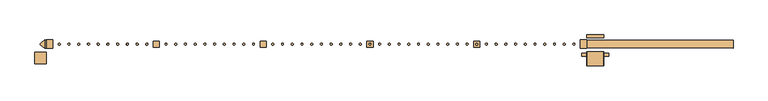
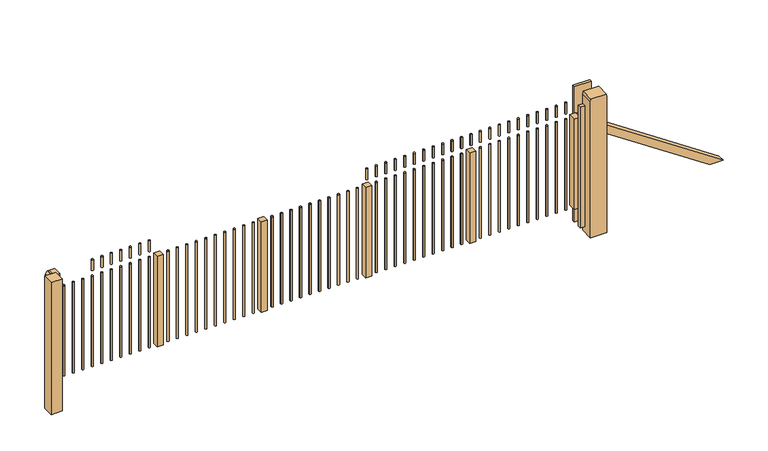
"""IFC4 building model written with IfcOpenShell, lengths in millimetres: door geometry, NLRS_90_DO_UN_schuifpoort met spijlen_gen_rsf : schuifpoort automatisch bxh 7000x1800-NP."""

from ifc_helpers import new_model, si_unit, point, frame, frame_2d, origin, place, context, project, spatial, polyline, circle_curve, trimmed, segment, composite_curve, outline, extrude, source, transform, mapped, element, save


def door_c2b4a2f6(model_context):
    return source(origin(), model_context, "Body", "SweptSolid", [
        extrude(outline(composite_curve([segment(trimmed(circle_curve(frame_2d((3299.5, 0.0)), 12.5), [point((3312.0, 0.0))], [point((3287.0, 0.0))], False, "CARTESIAN"), True, "CONTINUOUS"), segment(trimmed(circle_curve(frame_2d((3299.5, 0.0)), 12.5), [point((3287.0, 0.0))], [point((3312.0, 0.0))], False, "CARTESIAN"), True, "CONTINUOUS")], self_intersect=False)), frame((0.0, 0.0, 300.0), z_axis=(0.0, 0.0, 1.0), x_axis=(1.0, 0.0, 0.0)), (0.0, 0.0, 1.0), 1270.0),
        extrude(outline(composite_curve([segment(trimmed(circle_curve(frame_2d((3173.5, 0.0)), 12.5), [point((3186.0, 0.0))], [point((3161.0, 0.0))], False, "CARTESIAN"), True, "CONTINUOUS"), segment(trimmed(circle_curve(frame_2d((3173.5, 0.0)), 12.5), [point((3161.0, 0.0))], [point((3186.0, 0.0))], False, "CARTESIAN"), True, "CONTINUOUS")], self_intersect=False)), frame((0.0, 0.0, 300.0), z_axis=(0.0, 0.0, 1.0), x_axis=(1.0, 0.0, 0.0)), (0.0, 0.0, 1.0), 1270.0),
        extrude(outline(composite_curve([segment(trimmed(circle_curve(frame_2d((3047.5, 0.0)), 12.5), [point((3060.0, 0.0))], [point((3035.0, 0.0))], False, "CARTESIAN"), True, "CONTINUOUS"), segment(trimmed(circle_curve(frame_2d((3047.5, 0.0)), 12.5), [point((3035.0, 0.0))], [point((3060.0, 0.0))], False, "CARTESIAN"), True, "CONTINUOUS")], self_intersect=False)), frame((0.0, 0.0, 300.0), z_axis=(0.0, 0.0, 1.0), x_axis=(1.0, 0.0, 0.0)), (0.0, 0.0, 1.0), 1270.0),
        extrude(outline(composite_curve([segment(trimmed(circle_curve(frame_2d((2921.5, 0.0)), 12.5), [point((2934.0, 0.0))], [point((2909.0, 0.0))], False, "CARTESIAN"), True, "CONTINUOUS"), segment(trimmed(circle_curve(frame_2d((2921.5, 0.0)), 12.5), [point((2909.0, 0.0))], [point((2934.0, 0.0))], False, "CARTESIAN"), True, "CONTINUOUS")], self_intersect=False)), frame((0.0, 0.0, 300.0), z_axis=(0.0, 0.0, 1.0), x_axis=(1.0, 0.0, 0.0)), (0.0, 0.0, 1.0), 1270.0),
        extrude(outline(composite_curve([segment(trimmed(circle_curve(frame_2d((2795.5, 0.0)), 12.5), [point((2808.0, 0.0))], [point((2783.0, 0.0))], False, "CARTESIAN"), True, "CONTINUOUS"), segment(trimmed(circle_curve(frame_2d((2795.5, 0.0)), 12.5), [point((2783.0, 0.0))], [point((2808.0, 0.0))], False, "CARTESIAN"), True, "CONTINUOUS")], self_intersect=False)), frame((0.0, 0.0, 300.0), z_axis=(0.0, 0.0, 1.0), x_axis=(1.0, 0.0, 0.0)), (0.0, 0.0, 1.0), 1270.0),
        extrude(outline(composite_curve([segment(trimmed(circle_curve(frame_2d((2669.5, 0.0)), 12.5), [point((2682.0, 0.0))], [point((2657.0, 0.0))], False, "CARTESIAN"), True, "CONTINUOUS"), segment(trimmed(circle_curve(frame_2d((2669.5, 0.0)), 12.5), [point((2657.0, 0.0))], [point((2682.0, 0.0))], False, "CARTESIAN"), True, "CONTINUOUS")], self_intersect=False)), frame((0.0, 0.0, 300.0), z_axis=(0.0, 0.0, 1.0), x_axis=(1.0, 0.0, 0.0)), (0.0, 0.0, 1.0), 1270.0),
        extrude(outline(composite_curve([segment(trimmed(circle_curve(frame_2d((2543.5, 0.0)), 12.5), [point((2556.0, 0.0))], [point((2531.0, 0.0))], False, "CARTESIAN"), True, "CONTINUOUS"), segment(trimmed(circle_curve(frame_2d((2543.5, 0.0)), 12.5), [point((2531.0, 0.0))], [point((2556.0, 0.0))], False, "CARTESIAN"), True, "CONTINUOUS")], self_intersect=False)), frame((0.0, 0.0, 300.0), z_axis=(0.0, 0.0, 1.0), x_axis=(1.0, 0.0, 0.0)), (0.0, 0.0, 1.0), 1270.0),
        extrude(outline(composite_curve([segment(trimmed(circle_curve(frame_2d((2417.5, 0.0)), 12.5), [point((2430.0, 0.0))], [point((2405.0, 0.0))], False, "CARTESIAN"), True, "CONTINUOUS"), segment(trimmed(circle_curve(frame_2d((2417.5, 0.0)), 12.5), [point((2405.0, 0.0))], [point((2430.0, 0.0))], False, "CARTESIAN"), True, "CONTINUOUS")], self_intersect=False)), frame((0.0, 0.0, 300.0), z_axis=(0.0, 0.0, 1.0), x_axis=(1.0, 0.0, 0.0)), (0.0, 0.0, 1.0), 1270.0),
        extrude(outline(composite_curve([segment(trimmed(circle_curve(frame_2d((2291.5, 0.0)), 12.5), [point((2304.0, 0.0))], [point((2279.0, 0.0))], False, "CARTESIAN"), True, "CONTINUOUS"), segment(trimmed(circle_curve(frame_2d((2291.5, 0.0)), 12.5), [point((2279.0, 0.0))], [point((2304.0, 0.0))], False, "CARTESIAN"), True, "CONTINUOUS")], self_intersect=False)), frame((0.0, 0.0, 300.0), z_axis=(0.0, 0.0, 1.0), x_axis=(1.0, 0.0, 0.0)), (0.0, 0.0, 1.0), 1270.0),
        extrude(outline(composite_curve([segment(trimmed(circle_curve(frame_2d((2165.5, 0.0)), 12.5), [point((2178.0, 0.0))], [point((2153.0, 0.0))], False, "CARTESIAN"), True, "CONTINUOUS"), segment(trimmed(circle_curve(frame_2d((2165.5, 0.0)), 12.5), [point((2153.0, 0.0))], [point((2178.0, 0.0))], False, "CARTESIAN"), True, "CONTINUOUS")], self_intersect=False)), frame((0.0, 0.0, 300.0), z_axis=(0.0, 0.0, 1.0), x_axis=(1.0, 0.0, 0.0)), (0.0, 0.0, 1.0), 1270.0),
        extrude(outline(composite_curve([segment(trimmed(circle_curve(frame_2d((1915.5, 0.0)), 12.5), [point((1928.0, 0.0))], [point((1903.0, 0.0))], False, "CARTESIAN"), True, "CONTINUOUS"), segment(trimmed(circle_curve(frame_2d((1915.5, 0.0)), 12.5), [point((1903.0, 0.0))], [point((1928.0, 0.0))], False, "CARTESIAN"), True, "CONTINUOUS")], self_intersect=False)), frame((0.0, 0.0, 300.0), z_axis=(0.0, 0.0, 1.0), x_axis=(1.0, 0.0, 0.0)), (0.0, 0.0, 1.0), 1270.0),
        extrude(outline(composite_curve([segment(trimmed(circle_curve(frame_2d((1789.5, 0.0)), 12.5), [point((1802.0, 0.0))], [point((1777.0, 0.0))], False, "CARTESIAN"), True, "CONTINUOUS"), segment(trimmed(circle_curve(frame_2d((1789.5, 0.0)), 12.5), [point((1777.0, 0.0))], [point((1802.0, 0.0))], False, "CARTESIAN"), True, "CONTINUOUS")], self_intersect=False)), frame((0.0, 0.0, 300.0), z_axis=(0.0, 0.0, 1.0), x_axis=(1.0, 0.0, 0.0)), (0.0, 0.0, 1.0), 1270.0),
        extrude(outline(composite_curve([segment(trimmed(circle_curve(frame_2d((1663.5, 0.0)), 12.5), [point((1676.0, 0.0))], [point((1651.0, 0.0))], False, "CARTESIAN"), True, "CONTINUOUS"), segment(trimmed(circle_curve(frame_2d((1663.5, 0.0)), 12.5), [point((1651.0, 0.0))], [point((1676.0, 0.0))], False, "CARTESIAN"), True, "CONTINUOUS")], self_intersect=False)), frame((0.0, 0.0, 300.0), z_axis=(0.0, 0.0, 1.0), x_axis=(1.0, 0.0, 0.0)), (0.0, 0.0, 1.0), 1270.0),
        extrude(outline(composite_curve([segment(trimmed(circle_curve(frame_2d((1537.5, 0.0)), 12.5), [point((1550.0, 0.0))], [point((1525.0, 0.0))], False, "CARTESIAN"), True, "CONTINUOUS"), segment(trimmed(circle_curve(frame_2d((1537.5, 0.0)), 12.5), [point((1525.0, 0.0))], [point((1550.0, 0.0))], False, "CARTESIAN"), True, "CONTINUOUS")], self_intersect=False)), frame((0.0, 0.0, 300.0), z_axis=(0.0, 0.0, 1.0), x_axis=(1.0, 0.0, 0.0)), (0.0, 0.0, 1.0), 1270.0),
        extrude(outline(composite_curve([segment(trimmed(circle_curve(frame_2d((1411.5, 0.0)), 12.5), [point((1424.0, 0.0))], [point((1399.0, 0.0))], False, "CARTESIAN"), True, "CONTINUOUS"), segment(trimmed(circle_curve(frame_2d((1411.5, 0.0)), 12.5), [point((1399.0, 0.0))], [point((1424.0, 0.0))], False, "CARTESIAN"), True, "CONTINUOUS")], self_intersect=False)), frame((0.0, 0.0, 300.0), z_axis=(0.0, 0.0, 1.0), x_axis=(1.0, 0.0, 0.0)), (0.0, 0.0, 1.0), 1270.0),
        extrude(outline(composite_curve([segment(trimmed(circle_curve(frame_2d((1285.5, 0.0)), 12.5), [point((1298.0, 0.0))], [point((1273.0, 0.0))], False, "CARTESIAN"), True, "CONTINUOUS"), segment(trimmed(circle_curve(frame_2d((1285.5, 0.0)), 12.5), [point((1273.0, 0.0))], [point((1298.0, 0.0))], False, "CARTESIAN"), True, "CONTINUOUS")], self_intersect=False)), frame((0.0, 0.0, 300.0), z_axis=(0.0, 0.0, 1.0), x_axis=(1.0, 0.0, 0.0)), (0.0, 0.0, 1.0), 1270.0),
        extrude(outline(composite_curve([segment(trimmed(circle_curve(frame_2d((1159.5, 0.0)), 12.5), [point((1172.0, 0.0))], [point((1147.0, 0.0))], False, "CARTESIAN"), True, "CONTINUOUS"), segment(trimmed(circle_curve(frame_2d((1159.5, 0.0)), 12.5), [point((1147.0, 0.0))], [point((1172.0, 0.0))], False, "CARTESIAN"), True, "CONTINUOUS")], self_intersect=False)), frame((0.0, 0.0, 300.0), z_axis=(0.0, 0.0, 1.0), x_axis=(1.0, 0.0, 0.0)), (0.0, 0.0, 1.0), 1270.0),
        extrude(outline(composite_curve([segment(trimmed(circle_curve(frame_2d((1033.5, 0.0)), 12.5), [point((1046.0, 0.0))], [point((1021.0, 0.0))], False, "CARTESIAN"), True, "CONTINUOUS"), segment(trimmed(circle_curve(frame_2d((1033.5, 0.0)), 12.5), [point((1021.0, 0.0))], [point((1046.0, 0.0))], False, "CARTESIAN"), True, "CONTINUOUS")], self_intersect=False)), frame((0.0, 0.0, 300.0), z_axis=(0.0, 0.0, 1.0), x_axis=(1.0, 0.0, 0.0)), (0.0, 0.0, 1.0), 1270.0),
        extrude(outline(composite_curve([segment(trimmed(circle_curve(frame_2d((907.5, 0.0)), 12.5), [point((920.0, 0.0))], [point((895.0, 0.0))], False, "CARTESIAN"), True, "CONTINUOUS"), segment(trimmed(circle_curve(frame_2d((907.5, 0.0)), 12.5), [point((895.0, 0.0))], [point((920.0, 0.0))], False, "CARTESIAN"), True, "CONTINUOUS")], self_intersect=False)), frame((0.0, 0.0, 300.0), z_axis=(0.0, 0.0, 1.0), x_axis=(1.0, 0.0, 0.0)), (0.0, 0.0, 1.0), 1270.0),
        extrude(outline(composite_curve([segment(trimmed(circle_curve(frame_2d((781.5, 0.0)), 12.5), [point((794.0, 0.0))], [point((769.0, 0.0))], False, "CARTESIAN"), True, "CONTINUOUS"), segment(trimmed(circle_curve(frame_2d((781.5, 0.0)), 12.5), [point((769.0, 0.0))], [point((794.0, 0.0))], False, "CARTESIAN"), True, "CONTINUOUS")], self_intersect=False)), frame((0.0, 0.0, 300.0), z_axis=(0.0, 0.0, 1.0), x_axis=(1.0, 0.0, 0.0)), (0.0, 0.0, 1.0), 1270.0),
        extrude(outline(polyline([(3465.0, -158.5), (3400.0, -158.5), (3400.0, -118.5), (3465.0, -118.5), (3465.0, -158.5)])), frame((0.0, 0.0, 100.0), z_axis=(0.0, 0.0, 1.0), x_axis=(1.0, 0.0, 0.0)), (0.0, 0.0, 1.0), 1700.0),
        extrude(outline(polyline([(3685.0, -158.5), (3685.0, -118.5), (3750.0, -118.5), (3750.0, -158.5), (3685.0, -158.5)])), frame((0.0, 0.0, 100.0), z_axis=(0.0, 0.0, 1.0), x_axis=(1.0, 0.0, 0.0)), (0.0, 0.0, 1.0), 1700.0),
        extrude(outline(polyline([(3685.0, 84.5), (3465.0, 84.5), (3465.0, 119.5), (3685.0, 119.5), (3685.0, 84.5)])), frame((0.0, 0.0, 12.0), z_axis=(0.0, 0.0, 1.0), x_axis=(1.0, 0.0, 0.0)), (0.0, 0.0, 1.0), 1906.0),
        extrude(outline(polyline([(1918.0, 3465.0), (12.0, 3465.0), (12.0, 3685.0), (1918.0, 3685.0), (1960.0, 3677.5), (1960.0, 3472.5), (1918.0, 3465.0)])), frame((0.0, -280.5, 0.0), z_axis=(0.0, 1.0, 0.0), x_axis=(0.0, 0.0, 1.0)), (0.0, 0.0, 1.0), 180.0),
        extrude(outline(polyline([(2000.5, -40.0), (2000.5, 40.0), (2080.5, 40.0), (2080.5, -40.0), (2000.5, -40.0)])), frame((0.0, 0.0, 300.0), z_axis=(0.0, 0.0, 1.0), x_axis=(1.0, 0.0, 0.0)), (0.0, 0.0, 1.0), 1270.0),
        extrude(outline(polyline([(616.5, -40.0), (616.5, 40.0), (696.5, 40.0), (696.5, -40.0), (616.5, -40.0)])), frame((0.0, 0.0, 300.0), z_axis=(0.0, 0.0, 1.0), x_axis=(1.0, 0.0, 0.0)), (0.0, 0.0, 1.0), 1270.0),
        extrude(outline(polyline([(-767.5, -40.0), (-767.5, 40.0), (-687.5, 40.0), (-687.5, -40.0), (-767.5, -40.0)])), frame((0.0, 0.0, 300.0), z_axis=(0.0, 0.0, 1.0), x_axis=(1.0, 0.0, 0.0)), (0.0, 0.0, 1.0), 1270.0),
        extrude(outline(polyline([(-2151.5, -40.0), (-2151.5, 40.0), (-2071.5, 40.0), (-2071.5, -40.0), (-2151.5, -40.0)])), frame((0.0, 0.0, 300.0), z_axis=(0.0, 0.0, 1.0), x_axis=(1.0, 0.0, 0.0)), (0.0, 0.0, 1.0), 1270.0),
        extrude(outline(composite_curve([segment(trimmed(circle_curve(frame_2d((531.5, 0.0)), 12.5), [point((544.0, 0.0))], [point((519.0, 0.0))], False, "CARTESIAN"), True, "CONTINUOUS"), segment(trimmed(circle_curve(frame_2d((531.5, 0.0)), 12.5), [point((519.0, 0.0))], [point((544.0, 0.0))], False, "CARTESIAN"), True, "CONTINUOUS")], self_intersect=False)), frame((0.0, 0.0, 300.0), z_axis=(0.0, 0.0, 1.0), x_axis=(1.0, 0.0, 0.0)), (0.0, 0.0, 1.0), 1270.0),
        extrude(outline(composite_curve([segment(trimmed(circle_curve(frame_2d((405.5, 0.0)), 12.5), [point((418.0, 0.0))], [point((393.0, 0.0))], False, "CARTESIAN"), True, "CONTINUOUS"), segment(trimmed(circle_curve(frame_2d((405.5, 0.0)), 12.5), [point((393.0, 0.0))], [point((418.0, 0.0))], False, "CARTESIAN"), True, "CONTINUOUS")], self_intersect=False)), frame((0.0, 0.0, 300.0), z_axis=(0.0, 0.0, 1.0), x_axis=(1.0, 0.0, 0.0)), (0.0, 0.0, 1.0), 1270.0),
        extrude(outline(composite_curve([segment(trimmed(circle_curve(frame_2d((279.5, 0.0)), 12.5), [point((292.0, 0.0))], [point((267.0, 0.0))], False, "CARTESIAN"), True, "CONTINUOUS"), segment(trimmed(circle_curve(frame_2d((279.5, 0.0)), 12.5), [point((267.0, 0.0))], [point((292.0, 0.0))], False, "CARTESIAN"), True, "CONTINUOUS")], self_intersect=False)), frame((0.0, 0.0, 300.0), z_axis=(0.0, 0.0, 1.0), x_axis=(1.0, 0.0, 0.0)), (0.0, 0.0, 1.0), 1270.0),
        extrude(outline(composite_curve([segment(trimmed(circle_curve(frame_2d((153.5, 0.0)), 12.5), [point((166.0, 0.0))], [point((141.0, 0.0))], False, "CARTESIAN"), True, "CONTINUOUS"), segment(trimmed(circle_curve(frame_2d((153.5, 0.0)), 12.5), [point((141.0, 0.0))], [point((166.0, 0.0))], False, "CARTESIAN"), True, "CONTINUOUS")], self_intersect=False)), frame((0.0, 0.0, 300.0), z_axis=(0.0, 0.0, 1.0), x_axis=(1.0, 0.0, 0.0)), (0.0, 0.0, 1.0), 1270.0),
        extrude(outline(composite_curve([segment(trimmed(circle_curve(frame_2d((27.5, 0.0)), 12.5), [point((40.0, 0.0))], [point((15.0, 0.0))], False, "CARTESIAN"), True, "CONTINUOUS"), segment(trimmed(circle_curve(frame_2d((27.5, 0.0)), 12.5), [point((15.0, 0.0))], [point((40.0, 0.0))], False, "CARTESIAN"), True, "CONTINUOUS")], self_intersect=False)), frame((0.0, 0.0, 300.0), z_axis=(0.0, 0.0, 1.0), x_axis=(1.0, 0.0, 0.0)), (0.0, 0.0, 1.0), 1270.0),
        extrude(outline(composite_curve([segment(trimmed(circle_curve(frame_2d((-98.5, 0.0)), 12.5), [point((-86.0, 0.0))], [point((-111.0, 0.0))], False, "CARTESIAN"), True, "CONTINUOUS"), segment(trimmed(circle_curve(frame_2d((-98.5, 0.0)), 12.5), [point((-111.0, 0.0))], [point((-86.0, 0.0))], False, "CARTESIAN"), True, "CONTINUOUS")], self_intersect=False)), frame((0.0, 0.0, 300.0), z_axis=(0.0, 0.0, 1.0), x_axis=(1.0, 0.0, 0.0)), (0.0, 0.0, 1.0), 1270.0),
        extrude(outline(composite_curve([segment(trimmed(circle_curve(frame_2d((-224.5, 0.0)), 12.5), [point((-212.0, 0.0))], [point((-237.0, 0.0))], False, "CARTESIAN"), True, "CONTINUOUS"), segment(trimmed(circle_curve(frame_2d((-224.5, 0.0)), 12.5), [point((-237.0, 0.0))], [point((-212.0, 0.0))], False, "CARTESIAN"), True, "CONTINUOUS")], self_intersect=False)), frame((0.0, 0.0, 300.0), z_axis=(0.0, 0.0, 1.0), x_axis=(1.0, 0.0, 0.0)), (0.0, 0.0, 1.0), 1270.0),
        extrude(outline(composite_curve([segment(trimmed(circle_curve(frame_2d((-350.5, 0.0)), 12.5), [point((-338.0, 0.0))], [point((-363.0, 0.0))], False, "CARTESIAN"), True, "CONTINUOUS"), segment(trimmed(circle_curve(frame_2d((-350.5, 0.0)), 12.5), [point((-363.0, 0.0))], [point((-338.0, 0.0))], False, "CARTESIAN"), True, "CONTINUOUS")], self_intersect=False)), frame((0.0, 0.0, 300.0), z_axis=(0.0, 0.0, 1.0), x_axis=(1.0, 0.0, 0.0)), (0.0, 0.0, 1.0), 1270.0),
        extrude(outline(composite_curve([segment(trimmed(circle_curve(frame_2d((-476.5, 0.0)), 12.5), [point((-464.0, 0.0))], [point((-489.0, 0.0))], False, "CARTESIAN"), True, "CONTINUOUS"), segment(trimmed(circle_curve(frame_2d((-476.5, 0.0)), 12.5), [point((-489.0, 0.0))], [point((-464.0, 0.0))], False, "CARTESIAN"), True, "CONTINUOUS")], self_intersect=False)), frame((0.0, 0.0, 300.0), z_axis=(0.0, 0.0, 1.0), x_axis=(1.0, 0.0, 0.0)), (0.0, 0.0, 1.0), 1270.0),
        extrude(outline(composite_curve([segment(trimmed(circle_curve(frame_2d((-602.5, 0.0)), 12.5), [point((-590.0, 0.0))], [point((-615.0, 0.0))], False, "CARTESIAN"), True, "CONTINUOUS"), segment(trimmed(circle_curve(frame_2d((-602.5, 0.0)), 12.5), [point((-615.0, 0.0))], [point((-590.0, 0.0))], False, "CARTESIAN"), True, "CONTINUOUS")], self_intersect=False)), frame((0.0, 0.0, 300.0), z_axis=(0.0, 0.0, 1.0), x_axis=(1.0, 0.0, 0.0)), (0.0, 0.0, 1.0), 1270.0),
        extrude(outline(polyline([(300.0, 5362.0), (1570.0, 3464.5), (1449.6685917, 3464.5), (300.0, 5182.2135061), (300.0, 5362.0)])), frame((0.0, -50.0, 0.0), z_axis=(0.0, 1.0, 0.0), x_axis=(0.0, 0.0, 1.0)), (0.0, 0.0, 1.0), 100.0),
        extrude(outline(composite_curve([segment(trimmed(circle_curve(frame_2d((-852.5, 0.0)), 12.5), [point((-840.0, 0.0))], [point((-865.0, 0.0))], False, "CARTESIAN"), True, "CONTINUOUS"), segment(trimmed(circle_curve(frame_2d((-852.5, 0.0)), 12.5), [point((-865.0, 0.0))], [point((-840.0, 0.0))], False, "CARTESIAN"), True, "CONTINUOUS")], self_intersect=False)), frame((0.0, 0.0, 300.0), z_axis=(0.0, 0.0, 1.0), x_axis=(1.0, 0.0, 0.0)), (0.0, 0.0, 1.0), 1270.0),
        extrude(outline(composite_curve([segment(trimmed(circle_curve(frame_2d((-978.5, 0.0)), 12.5), [point((-966.0, 0.0))], [point((-991.0, 0.0))], False, "CARTESIAN"), True, "CONTINUOUS"), segment(trimmed(circle_curve(frame_2d((-978.5, 0.0)), 12.5), [point((-991.0, 0.0))], [point((-966.0, 0.0))], False, "CARTESIAN"), True, "CONTINUOUS")], self_intersect=False)), frame((0.0, 0.0, 300.0), z_axis=(0.0, 0.0, 1.0), x_axis=(1.0, 0.0, 0.0)), (0.0, 0.0, 1.0), 1270.0),
        extrude(outline(composite_curve([segment(trimmed(circle_curve(frame_2d((-1104.5, 0.0)), 12.5), [point((-1092.0, 0.0))], [point((-1117.0, 0.0))], False, "CARTESIAN"), True, "CONTINUOUS"), segment(trimmed(circle_curve(frame_2d((-1104.5, 0.0)), 12.5), [point((-1117.0, 0.0))], [point((-1092.0, 0.0))], False, "CARTESIAN"), True, "CONTINUOUS")], self_intersect=False)), frame((0.0, 0.0, 300.0), z_axis=(0.0, 0.0, 1.0), x_axis=(1.0, 0.0, 0.0)), (0.0, 0.0, 1.0), 1270.0),
        extrude(outline(composite_curve([segment(trimmed(circle_curve(frame_2d((-1230.5, 0.0)), 12.5), [point((-1218.0, 0.0))], [point((-1243.0, 0.0))], False, "CARTESIAN"), True, "CONTINUOUS"), segment(trimmed(circle_curve(frame_2d((-1230.5, 0.0)), 12.5), [point((-1243.0, 0.0))], [point((-1218.0, 0.0))], False, "CARTESIAN"), True, "CONTINUOUS")], self_intersect=False)), frame((0.0, 0.0, 300.0), z_axis=(0.0, 0.0, 1.0), x_axis=(1.0, 0.0, 0.0)), (0.0, 0.0, 1.0), 1270.0),
        extrude(outline(composite_curve([segment(trimmed(circle_curve(frame_2d((-1356.5, 0.0)), 12.5), [point((-1344.0, 0.0))], [point((-1369.0, 0.0))], False, "CARTESIAN"), True, "CONTINUOUS"), segment(trimmed(circle_curve(frame_2d((-1356.5, 0.0)), 12.5), [point((-1369.0, 0.0))], [point((-1344.0, 0.0))], False, "CARTESIAN"), True, "CONTINUOUS")], self_intersect=False)), frame((0.0, 0.0, 300.0), z_axis=(0.0, 0.0, 1.0), x_axis=(1.0, 0.0, 0.0)), (0.0, 0.0, 1.0), 1270.0),
        extrude(outline(composite_curve([segment(trimmed(circle_curve(frame_2d((-1482.5, 0.0)), 12.5), [point((-1470.0, 0.0))], [point((-1495.0, 0.0))], False, "CARTESIAN"), True, "CONTINUOUS"), segment(trimmed(circle_curve(frame_2d((-1482.5, 0.0)), 12.5), [point((-1495.0, 0.0))], [point((-1470.0, 0.0))], False, "CARTESIAN"), True, "CONTINUOUS")], self_intersect=False)), frame((0.0, 0.0, 300.0), z_axis=(0.0, 0.0, 1.0), x_axis=(1.0, 0.0, 0.0)), (0.0, 0.0, 1.0), 1270.0),
        extrude(outline(composite_curve([segment(trimmed(circle_curve(frame_2d((-1608.5, 0.0)), 12.5), [point((-1596.0, 0.0))], [point((-1621.0, 0.0))], False, "CARTESIAN"), True, "CONTINUOUS"), segment(trimmed(circle_curve(frame_2d((-1608.5, 0.0)), 12.5), [point((-1621.0, 0.0))], [point((-1596.0, 0.0))], False, "CARTESIAN"), True, "CONTINUOUS")], self_intersect=False)), frame((0.0, 0.0, 300.0), z_axis=(0.0, 0.0, 1.0), x_axis=(1.0, 0.0, 0.0)), (0.0, 0.0, 1.0), 1270.0),
        extrude(outline(composite_curve([segment(trimmed(circle_curve(frame_2d((-1734.5, 0.0)), 12.5), [point((-1722.0, 0.0))], [point((-1747.0, 0.0))], False, "CARTESIAN"), True, "CONTINUOUS"), segment(trimmed(circle_curve(frame_2d((-1734.5, 0.0)), 12.5), [point((-1747.0, 0.0))], [point((-1722.0, 0.0))], False, "CARTESIAN"), True, "CONTINUOUS")], self_intersect=False)), frame((0.0, 0.0, 300.0), z_axis=(0.0, 0.0, 1.0), x_axis=(1.0, 0.0, 0.0)), (0.0, 0.0, 1.0), 1270.0),
        extrude(outline(composite_curve([segment(trimmed(circle_curve(frame_2d((-1860.5, 0.0)), 12.5), [point((-1848.0, 0.0))], [point((-1873.0, 0.0))], False, "CARTESIAN"), True, "CONTINUOUS"), segment(trimmed(circle_curve(frame_2d((-1860.5, 0.0)), 12.5), [point((-1873.0, 0.0))], [point((-1848.0, 0.0))], False, "CARTESIAN"), True, "CONTINUOUS")], self_intersect=False)), frame((0.0, 0.0, 300.0), z_axis=(0.0, 0.0, 1.0), x_axis=(1.0, 0.0, 0.0)), (0.0, 0.0, 1.0), 1270.0),
        extrude(outline(composite_curve([segment(trimmed(circle_curve(frame_2d((-1986.5, 0.0)), 12.5), [point((-1974.0, 0.0))], [point((-1999.0, 0.0))], False, "CARTESIAN"), True, "CONTINUOUS"), segment(trimmed(circle_curve(frame_2d((-1986.5, 0.0)), 12.5), [point((-1999.0, 0.0))], [point((-1974.0, 0.0))], False, "CARTESIAN"), True, "CONTINUOUS")], self_intersect=False)), frame((0.0, 0.0, 300.0), z_axis=(0.0, 0.0, 1.0), x_axis=(1.0, 0.0, 0.0)), (0.0, 0.0, 1.0), 1270.0),
        extrude(outline(composite_curve([segment(trimmed(circle_curve(frame_2d((-2236.0, 0.0)), 12.5), [point((-2223.5, 0.0))], [point((-2248.5, 0.0))], False, "CARTESIAN"), True, "CONTINUOUS"), segment(trimmed(circle_curve(frame_2d((-2236.0, 0.0)), 12.5), [point((-2248.5, 0.0))], [point((-2223.5, 0.0))], False, "CARTESIAN"), True, "CONTINUOUS")], self_intersect=False)), frame((0.0, 0.0, 300.0), z_axis=(0.0, 0.0, 1.0), x_axis=(1.0, 0.0, 0.0)), (0.0, 0.0, 1.0), 1270.0),
        extrude(outline(composite_curve([segment(trimmed(circle_curve(frame_2d((-2362.0, 0.0)), 12.5), [point((-2349.5, 0.0))], [point((-2374.5, 0.0))], False, "CARTESIAN"), True, "CONTINUOUS"), segment(trimmed(circle_curve(frame_2d((-2362.0, 0.0)), 12.5), [point((-2374.5, 0.0))], [point((-2349.5, 0.0))], False, "CARTESIAN"), True, "CONTINUOUS")], self_intersect=False)), frame((0.0, 0.0, 300.0), z_axis=(0.0, 0.0, 1.0), x_axis=(1.0, 0.0, 0.0)), (0.0, 0.0, 1.0), 1270.0),
        extrude(outline(composite_curve([segment(trimmed(circle_curve(frame_2d((-2488.0, 0.0)), 12.5), [point((-2475.5, 0.0))], [point((-2500.5, 0.0))], False, "CARTESIAN"), True, "CONTINUOUS"), segment(trimmed(circle_curve(frame_2d((-2488.0, 0.0)), 12.5), [point((-2500.5, 0.0))], [point((-2475.5, 0.0))], False, "CARTESIAN"), True, "CONTINUOUS")], self_intersect=False)), frame((0.0, 0.0, 300.0), z_axis=(0.0, 0.0, 1.0), x_axis=(1.0, 0.0, 0.0)), (0.0, 0.0, 1.0), 1270.0),
        extrude(outline(composite_curve([segment(trimmed(circle_curve(frame_2d((-2614.0, 0.0)), 12.5), [point((-2601.5, 0.0))], [point((-2626.5, 0.0))], False, "CARTESIAN"), True, "CONTINUOUS"), segment(trimmed(circle_curve(frame_2d((-2614.0, 0.0)), 12.5), [point((-2626.5, 0.0))], [point((-2601.5, 0.0))], False, "CARTESIAN"), True, "CONTINUOUS")], self_intersect=False)), frame((0.0, 0.0, 300.0), z_axis=(0.0, 0.0, 1.0), x_axis=(1.0, 0.0, 0.0)), (0.0, 0.0, 1.0), 1270.0),
        extrude(outline(composite_curve([segment(trimmed(circle_curve(frame_2d((-2740.0, 0.0)), 12.5), [point((-2727.5, 0.0))], [point((-2752.5, 0.0))], False, "CARTESIAN"), True, "CONTINUOUS"), segment(trimmed(circle_curve(frame_2d((-2740.0, 0.0)), 12.5), [point((-2752.5, 0.0))], [point((-2727.5, 0.0))], False, "CARTESIAN"), True, "CONTINUOUS")], self_intersect=False)), frame((0.0, 0.0, 300.0), z_axis=(0.0, 0.0, 1.0), x_axis=(1.0, 0.0, 0.0)), (0.0, 0.0, 1.0), 1270.0),
        extrude(outline(composite_curve([segment(trimmed(circle_curve(frame_2d((-2866.0, 0.0)), 12.5), [point((-2853.5, 0.0))], [point((-2878.5, 0.0))], False, "CARTESIAN"), True, "CONTINUOUS"), segment(trimmed(circle_curve(frame_2d((-2866.0, 0.0)), 12.5), [point((-2878.5, 0.0))], [point((-2853.5, 0.0))], False, "CARTESIAN"), True, "CONTINUOUS")], self_intersect=False)), frame((0.0, 0.0, 300.0), z_axis=(0.0, 0.0, 1.0), x_axis=(1.0, 0.0, 0.0)), (0.0, 0.0, 1.0), 1270.0),
        extrude(outline(composite_curve([segment(trimmed(circle_curve(frame_2d((-2992.0, 0.0)), 12.5), [point((-2979.5, 0.0))], [point((-3004.5, 0.0))], False, "CARTESIAN"), True, "CONTINUOUS"), segment(trimmed(circle_curve(frame_2d((-2992.0, 0.0)), 12.5), [point((-3004.5, 0.0))], [point((-2979.5, 0.0))], False, "CARTESIAN"), True, "CONTINUOUS")], self_intersect=False)), frame((0.0, 0.0, 300.0), z_axis=(0.0, 0.0, 1.0), x_axis=(1.0, 0.0, 0.0)), (0.0, 0.0, 1.0), 1270.0),
        extrude(outline(composite_curve([segment(trimmed(circle_curve(frame_2d((-3118.0, 0.0)), 12.5), [point((-3105.5, 0.0))], [point((-3130.5, 0.0))], False, "CARTESIAN"), True, "CONTINUOUS"), segment(trimmed(circle_curve(frame_2d((-3118.0, 0.0)), 12.5), [point((-3130.5, 0.0))], [point((-3105.5, 0.0))], False, "CARTESIAN"), True, "CONTINUOUS")], self_intersect=False)), frame((0.0, 0.0, 300.0), z_axis=(0.0, 0.0, 1.0), x_axis=(1.0, 0.0, 0.0)), (0.0, 0.0, 1.0), 1270.0),
        extrude(outline(composite_curve([segment(trimmed(circle_curve(frame_2d((-3244.0, 0.0)), 12.5), [point((-3231.5, 0.0))], [point((-3256.5, 0.0))], False, "CARTESIAN"), True, "CONTINUOUS"), segment(trimmed(circle_curve(frame_2d((-3244.0, 0.0)), 12.5), [point((-3256.5, 0.0))], [point((-3231.5, 0.0))], False, "CARTESIAN"), True, "CONTINUOUS")], self_intersect=False)), frame((0.0, 0.0, 300.0), z_axis=(0.0, 0.0, 1.0), x_axis=(1.0, 0.0, 0.0)), (0.0, 0.0, 1.0), 1270.0),
        extrude(outline(composite_curve([segment(trimmed(circle_curve(frame_2d((-3370.0, 0.0)), 12.5), [point((-3357.5, 0.0))], [point((-3382.5, 0.0))], False, "CARTESIAN"), True, "CONTINUOUS"), segment(trimmed(circle_curve(frame_2d((-3370.0, 0.0)), 12.5), [point((-3382.5, 0.0))], [point((-3357.5, 0.0))], False, "CARTESIAN"), True, "CONTINUOUS")], self_intersect=False)), frame((0.0, 0.0, 300.0), z_axis=(0.0, 0.0, 1.0), x_axis=(1.0, 0.0, 0.0)), (0.0, 0.0, 1.0), 1270.0),
        extrude(outline(composite_curve([segment(trimmed(circle_curve(frame_2d((-3557.5075149, 52.6282432)), 1.9937769), [point((-3558.78125, 54.1621094))], [point((-3555.53125, 52.8919162))], False, "CARTESIAN"), True, "CONTINUOUS"), segment(polyline([(-3555.53125, 52.8919162), (-3555.53125, -52.2876138)]), True, "CONTINUOUS"), segment(trimmed(circle_curve(frame_2d((-3557.4950392, -52.6395691)), 1.9950791), [point((-3555.53125, -52.2876138))], [point((-3558.765625, -54.1777344))], False, "CARTESIAN"), True, "CONTINUOUS"), segment(polyline([(-3558.765625, -54.1777344), (-3609.625, -11.4902343)]), True, "CONTINUOUS"), segment(trimmed(circle_curve(frame_2d((-3600.0040885, 0.0)), 14.9862412), [point((-3609.625, -11.4902343))], [point((-3609.625, 11.4902343))], False, "CARTESIAN"), True, "CONTINUOUS"), segment(polyline([(-3609.625, 11.4902343), (-3558.78125, 54.1621094)]), True, "CONTINUOUS")], self_intersect=False)), frame((0.0, 0.0, 100.0), z_axis=(0.0, 0.0, 1.0), x_axis=(1.0, 0.0, 0.0)), (0.0, 0.0, 1.0), 1700.0),
        extrude(outline(polyline([(-3535.5, -52.8125), (-3555.53125, -52.8125), (-3555.53125, 52.8125), (-3535.5, 52.8125), (-3535.5, -52.8125)])), frame((0.0, 0.0, 100.0), z_axis=(0.0, 0.0, 1.0), x_axis=(1.0, 0.0, 0.0)), (0.0, 0.0, 1.0), 1700.0),
        extrude(outline(polyline([(-3535.0, -255.5), (-3685.0, -255.5), (-3685.0, -105.5), (-3535.0, -105.5), (-3535.0, -255.5)])), frame((0.0, 0.0, 12.0), z_axis=(0.0, 0.0, 1.0), x_axis=(1.0, 0.0, 0.0)), (0.0, 0.0, 1.0), 1861.0),
        extrude(outline(polyline([(3464.5, -55.0), (3384.5, -55.0), (3384.5, 55.0), (3464.5, 55.0), (3464.5, -55.0)])), frame((0.0, 0.0, 300.0), z_axis=(0.0, 0.0, 1.0), x_axis=(1.0, 0.0, 0.0)), (0.0, 0.0, 1.0), 1270.0),
        extrude(outline(polyline([(-3455.5, -55.0), (-3535.5, -55.0), (-3535.5, 55.0), (-3455.5, 55.0), (-3455.5, -55.0)])), frame((0.0, 0.0, 300.0), z_axis=(0.0, 0.0, 1.0), x_axis=(1.0, 0.0, 0.0)), (0.0, 0.0, 1.0), 1500.0),
        extrude(outline(composite_curve([segment(trimmed(circle_curve(frame_2d((3299.5, 0.0)), 12.5), [point((3312.0, 0.0))], [point((3287.0, 0.0))], False, "CARTESIAN"), True, "CONTINUOUS"), segment(trimmed(circle_curve(frame_2d((3299.5, 0.0)), 12.5), [point((3287.0, 0.0))], [point((3312.0, 0.0))], False, "CARTESIAN"), True, "CONTINUOUS")], self_intersect=False)), frame((0.0, 0.0, 1650.0), z_axis=(0.0, 0.0, 1.0), x_axis=(1.0, 0.0, 0.0)), (0.0, 0.0, 1.0), 150.0),
        extrude(outline(composite_curve([segment(trimmed(circle_curve(frame_2d((3173.5, 0.0)), 12.5), [point((3186.0, 0.0))], [point((3161.0, 0.0))], False, "CARTESIAN"), True, "CONTINUOUS"), segment(trimmed(circle_curve(frame_2d((3173.5, 0.0)), 12.5), [point((3161.0, 0.0))], [point((3186.0, 0.0))], False, "CARTESIAN"), True, "CONTINUOUS")], self_intersect=False)), frame((0.0, 0.0, 1650.0), z_axis=(0.0, 0.0, 1.0), x_axis=(1.0, 0.0, 0.0)), (0.0, 0.0, 1.0), 150.0),
        extrude(outline(composite_curve([segment(trimmed(circle_curve(frame_2d((3047.5, 0.0)), 12.5), [point((3060.0, 0.0))], [point((3035.0, 0.0))], False, "CARTESIAN"), True, "CONTINUOUS"), segment(trimmed(circle_curve(frame_2d((3047.5, 0.0)), 12.5), [point((3035.0, 0.0))], [point((3060.0, 0.0))], False, "CARTESIAN"), True, "CONTINUOUS")], self_intersect=False)), frame((0.0, 0.0, 1650.0), z_axis=(0.0, 0.0, 1.0), x_axis=(1.0, 0.0, 0.0)), (0.0, 0.0, 1.0), 150.0),
        extrude(outline(composite_curve([segment(trimmed(circle_curve(frame_2d((2921.5, 0.0)), 12.5), [point((2934.0, 0.0))], [point((2909.0, 0.0))], False, "CARTESIAN"), True, "CONTINUOUS"), segment(trimmed(circle_curve(frame_2d((2921.5, 0.0)), 12.5), [point((2909.0, 0.0))], [point((2934.0, 0.0))], False, "CARTESIAN"), True, "CONTINUOUS")], self_intersect=False)), frame((0.0, 0.0, 1650.0), z_axis=(0.0, 0.0, 1.0), x_axis=(1.0, 0.0, 0.0)), (0.0, 0.0, 1.0), 150.0),
        extrude(outline(composite_curve([segment(trimmed(circle_curve(frame_2d((2795.5, 0.0)), 12.5), [point((2808.0, 0.0))], [point((2783.0, 0.0))], False, "CARTESIAN"), True, "CONTINUOUS"), segment(trimmed(circle_curve(frame_2d((2795.5, 0.0)), 12.5), [point((2783.0, 0.0))], [point((2808.0, 0.0))], False, "CARTESIAN"), True, "CONTINUOUS")], self_intersect=False)), frame((0.0, 0.0, 1650.0), z_axis=(0.0, 0.0, 1.0), x_axis=(1.0, 0.0, 0.0)), (0.0, 0.0, 1.0), 150.0),
        extrude(outline(composite_curve([segment(trimmed(circle_curve(frame_2d((2669.5, 0.0)), 12.5), [point((2682.0, 0.0))], [point((2657.0, 0.0))], False, "CARTESIAN"), True, "CONTINUOUS"), segment(trimmed(circle_curve(frame_2d((2669.5, 0.0)), 12.5), [point((2657.0, 0.0))], [point((2682.0, 0.0))], False, "CARTESIAN"), True, "CONTINUOUS")], self_intersect=False)), frame((0.0, 0.0, 1650.0), z_axis=(0.0, 0.0, 1.0), x_axis=(1.0, 0.0, 0.0)), (0.0, 0.0, 1.0), 150.0),
        extrude(outline(composite_curve([segment(trimmed(circle_curve(frame_2d((2543.5, 0.0)), 12.5), [point((2556.0, 0.0))], [point((2531.0, 0.0))], False, "CARTESIAN"), True, "CONTINUOUS"), segment(trimmed(circle_curve(frame_2d((2543.5, 0.0)), 12.5), [point((2531.0, 0.0))], [point((2556.0, 0.0))], False, "CARTESIAN"), True, "CONTINUOUS")], self_intersect=False)), frame((0.0, 0.0, 1650.0), z_axis=(0.0, 0.0, 1.0), x_axis=(1.0, 0.0, 0.0)), (0.0, 0.0, 1.0), 150.0),
        extrude(outline(composite_curve([segment(trimmed(circle_curve(frame_2d((2417.5, 0.0)), 12.5), [point((2430.0, 0.0))], [point((2405.0, 0.0))], False, "CARTESIAN"), True, "CONTINUOUS"), segment(trimmed(circle_curve(frame_2d((2417.5, 0.0)), 12.5), [point((2405.0, 0.0))], [point((2430.0, 0.0))], False, "CARTESIAN"), True, "CONTINUOUS")], self_intersect=False)), frame((0.0, 0.0, 1650.0), z_axis=(0.0, 0.0, 1.0), x_axis=(1.0, 0.0, 0.0)), (0.0, 0.0, 1.0), 150.0),
        extrude(outline(composite_curve([segment(trimmed(circle_curve(frame_2d((2291.5, 0.0)), 12.5), [point((2304.0, 0.0))], [point((2279.0, 0.0))], False, "CARTESIAN"), True, "CONTINUOUS"), segment(trimmed(circle_curve(frame_2d((2291.5, 0.0)), 12.5), [point((2279.0, 0.0))], [point((2304.0, 0.0))], False, "CARTESIAN"), True, "CONTINUOUS")], self_intersect=False)), frame((0.0, 0.0, 1650.0), z_axis=(0.0, 0.0, 1.0), x_axis=(1.0, 0.0, 0.0)), (0.0, 0.0, 1.0), 150.0),
        extrude(outline(composite_curve([segment(trimmed(circle_curve(frame_2d((2165.5, 0.0)), 12.5), [point((2178.0, 0.0))], [point((2153.0, 0.0))], False, "CARTESIAN"), True, "CONTINUOUS"), segment(trimmed(circle_curve(frame_2d((2165.5, 0.0)), 12.5), [point((2153.0, 0.0))], [point((2178.0, 0.0))], False, "CARTESIAN"), True, "CONTINUOUS")], self_intersect=False)), frame((0.0, 0.0, 1650.0), z_axis=(0.0, 0.0, 1.0), x_axis=(1.0, 0.0, 0.0)), (0.0, 0.0, 1.0), 150.0),
        extrude(outline(composite_curve([segment(trimmed(circle_curve(frame_2d((2040.5, 0.0)), 12.5), [point((2053.0, 0.0))], [point((2028.0, 0.0))], False, "CARTESIAN"), True, "CONTINUOUS"), segment(trimmed(circle_curve(frame_2d((2040.5, 0.0)), 12.5), [point((2028.0, 0.0))], [point((2053.0, 0.0))], False, "CARTESIAN"), True, "CONTINUOUS")], self_intersect=False)), frame((0.0, 0.0, 1650.0), z_axis=(0.0, 0.0, 1.0), x_axis=(1.0, 0.0, 0.0)), (0.0, 0.0, 1.0), 150.0),
        extrude(outline(composite_curve([segment(trimmed(circle_curve(frame_2d((656.5, 0.0)), 12.5), [point((669.0, 0.0))], [point((644.0, 0.0))], False, "CARTESIAN"), True, "CONTINUOUS"), segment(trimmed(circle_curve(frame_2d((656.5, 0.0)), 12.5), [point((644.0, 0.0))], [point((669.0, 0.0))], False, "CARTESIAN"), True, "CONTINUOUS")], self_intersect=False)), frame((0.0, 0.0, 1650.0), z_axis=(0.0, 0.0, 1.0), x_axis=(1.0, 0.0, 0.0)), (0.0, 0.0, 1.0), 150.0),
        extrude(outline(composite_curve([segment(trimmed(circle_curve(frame_2d((1915.5, 0.0)), 12.5), [point((1928.0, 0.0))], [point((1903.0, 0.0))], False, "CARTESIAN"), True, "CONTINUOUS"), segment(trimmed(circle_curve(frame_2d((1915.5, 0.0)), 12.5), [point((1903.0, 0.0))], [point((1928.0, 0.0))], False, "CARTESIAN"), True, "CONTINUOUS")], self_intersect=False)), frame((0.0, 0.0, 1650.0), z_axis=(0.0, 0.0, 1.0), x_axis=(1.0, 0.0, 0.0)), (0.0, 0.0, 1.0), 150.0),
        extrude(outline(composite_curve([segment(trimmed(circle_curve(frame_2d((1789.5, 0.0)), 12.5), [point((1802.0, 0.0))], [point((1777.0, 0.0))], False, "CARTESIAN"), True, "CONTINUOUS"), segment(trimmed(circle_curve(frame_2d((1789.5, 0.0)), 12.5), [point((1777.0, 0.0))], [point((1802.0, 0.0))], False, "CARTESIAN"), True, "CONTINUOUS")], self_intersect=False)), frame((0.0, 0.0, 1650.0), z_axis=(0.0, 0.0, 1.0), x_axis=(1.0, 0.0, 0.0)), (0.0, 0.0, 1.0), 150.0),
        extrude(outline(composite_curve([segment(trimmed(circle_curve(frame_2d((1663.5, 0.0)), 12.5), [point((1676.0, 0.0))], [point((1651.0, 0.0))], False, "CARTESIAN"), True, "CONTINUOUS"), segment(trimmed(circle_curve(frame_2d((1663.5, 0.0)), 12.5), [point((1651.0, 0.0))], [point((1676.0, 0.0))], False, "CARTESIAN"), True, "CONTINUOUS")], self_intersect=False)), frame((0.0, 0.0, 1650.0), z_axis=(0.0, 0.0, 1.0), x_axis=(1.0, 0.0, 0.0)), (0.0, 0.0, 1.0), 150.0),
        extrude(outline(composite_curve([segment(trimmed(circle_curve(frame_2d((1537.5, 0.0)), 12.5), [point((1550.0, 0.0))], [point((1525.0, 0.0))], False, "CARTESIAN"), True, "CONTINUOUS"), segment(trimmed(circle_curve(frame_2d((1537.5, 0.0)), 12.5), [point((1525.0, 0.0))], [point((1550.0, 0.0))], False, "CARTESIAN"), True, "CONTINUOUS")], self_intersect=False)), frame((0.0, 0.0, 1650.0), z_axis=(0.0, 0.0, 1.0), x_axis=(1.0, 0.0, 0.0)), (0.0, 0.0, 1.0), 150.0),
        extrude(outline(composite_curve([segment(trimmed(circle_curve(frame_2d((1411.5, 0.0)), 12.5), [point((1424.0, 0.0))], [point((1399.0, 0.0))], False, "CARTESIAN"), True, "CONTINUOUS"), segment(trimmed(circle_curve(frame_2d((1411.5, 0.0)), 12.5), [point((1399.0, 0.0))], [point((1424.0, 0.0))], False, "CARTESIAN"), True, "CONTINUOUS")], self_intersect=False)), frame((0.0, 0.0, 1650.0), z_axis=(0.0, 0.0, 1.0), x_axis=(1.0, 0.0, 0.0)), (0.0, 0.0, 1.0), 150.0),
        extrude(outline(composite_curve([segment(trimmed(circle_curve(frame_2d((1285.5, 0.0)), 12.5), [point((1298.0, 0.0))], [point((1273.0, 0.0))], False, "CARTESIAN"), True, "CONTINUOUS"), segment(trimmed(circle_curve(frame_2d((1285.5, 0.0)), 12.5), [point((1273.0, 0.0))], [point((1298.0, 0.0))], False, "CARTESIAN"), True, "CONTINUOUS")], self_intersect=False)), frame((0.0, 0.0, 1650.0), z_axis=(0.0, 0.0, 1.0), x_axis=(1.0, 0.0, 0.0)), (0.0, 0.0, 1.0), 150.0),
        extrude(outline(composite_curve([segment(trimmed(circle_curve(frame_2d((1159.5, 0.0)), 12.5), [point((1172.0, 0.0))], [point((1147.0, 0.0))], False, "CARTESIAN"), True, "CONTINUOUS"), segment(trimmed(circle_curve(frame_2d((1159.5, 0.0)), 12.5), [point((1147.0, 0.0))], [point((1172.0, 0.0))], False, "CARTESIAN"), True, "CONTINUOUS")], self_intersect=False)), frame((0.0, 0.0, 1650.0), z_axis=(0.0, 0.0, 1.0), x_axis=(1.0, 0.0, 0.0)), (0.0, 0.0, 1.0), 150.0),
        extrude(outline(composite_curve([segment(trimmed(circle_curve(frame_2d((1033.5, 0.0)), 12.5), [point((1046.0, 0.0))], [point((1021.0, 0.0))], False, "CARTESIAN"), True, "CONTINUOUS"), segment(trimmed(circle_curve(frame_2d((1033.5, 0.0)), 12.5), [point((1021.0, 0.0))], [point((1046.0, 0.0))], False, "CARTESIAN"), True, "CONTINUOUS")], self_intersect=False)), frame((0.0, 0.0, 1650.0), z_axis=(0.0, 0.0, 1.0), x_axis=(1.0, 0.0, 0.0)), (0.0, 0.0, 1.0), 150.0),
        extrude(outline(composite_curve([segment(trimmed(circle_curve(frame_2d((907.5, 0.0)), 12.5), [point((920.0, 0.0))], [point((895.0, 0.0))], False, "CARTESIAN"), True, "CONTINUOUS"), segment(trimmed(circle_curve(frame_2d((907.5, 0.0)), 12.5), [point((895.0, 0.0))], [point((920.0, 0.0))], False, "CARTESIAN"), True, "CONTINUOUS")], self_intersect=False)), frame((0.0, 0.0, 1650.0), z_axis=(0.0, 0.0, 1.0), x_axis=(1.0, 0.0, 0.0)), (0.0, 0.0, 1.0), 150.0),
        extrude(outline(composite_curve([segment(trimmed(circle_curve(frame_2d((781.5, 0.0)), 12.5), [point((794.0, 0.0))], [point((769.0, 0.0))], False, "CARTESIAN"), True, "CONTINUOUS"), segment(trimmed(circle_curve(frame_2d((781.5, 0.0)), 12.5), [point((769.0, 0.0))], [point((794.0, 0.0))], False, "CARTESIAN"), True, "CONTINUOUS")], self_intersect=False)), frame((0.0, 0.0, 1650.0), z_axis=(0.0, 0.0, 1.0), x_axis=(1.0, 0.0, 0.0)), (0.0, 0.0, 1.0), 150.0),
        extrude(outline(composite_curve([segment(trimmed(circle_curve(frame_2d((-2233.5, 0.0)), 12.5), [point((-2221.0, 0.0))], [point((-2246.0, 0.0))], False, "CARTESIAN"), True, "CONTINUOUS"), segment(trimmed(circle_curve(frame_2d((-2233.5, 0.0)), 12.5), [point((-2246.0, 0.0))], [point((-2221.0, 0.0))], False, "CARTESIAN"), True, "CONTINUOUS")], self_intersect=False)), frame((0.0, 0.0, 1650.0), z_axis=(0.0, 0.0, 1.0), x_axis=(1.0, 0.0, 0.0)), (0.0, 0.0, 1.0), 150.0),
        extrude(outline(composite_curve([segment(trimmed(circle_curve(frame_2d((-2359.5, 0.0)), 12.5), [point((-2347.0, 0.0))], [point((-2372.0, 0.0))], False, "CARTESIAN"), True, "CONTINUOUS"), segment(trimmed(circle_curve(frame_2d((-2359.5, 0.0)), 12.5), [point((-2372.0, 0.0))], [point((-2347.0, 0.0))], False, "CARTESIAN"), True, "CONTINUOUS")], self_intersect=False)), frame((0.0, 0.0, 1650.0), z_axis=(0.0, 0.0, 1.0), x_axis=(1.0, 0.0, 0.0)), (0.0, 0.0, 1.0), 150.0),
        extrude(outline(composite_curve([segment(trimmed(circle_curve(frame_2d((-2485.5, 0.0)), 12.5), [point((-2473.0, 0.0))], [point((-2498.0, 0.0))], False, "CARTESIAN"), True, "CONTINUOUS"), segment(trimmed(circle_curve(frame_2d((-2485.5, 0.0)), 12.5), [point((-2498.0, 0.0))], [point((-2473.0, 0.0))], False, "CARTESIAN"), True, "CONTINUOUS")], self_intersect=False)), frame((0.0, 0.0, 1650.0), z_axis=(0.0, 0.0, 1.0), x_axis=(1.0, 0.0, 0.0)), (0.0, 0.0, 1.0), 150.0),
        extrude(outline(composite_curve([segment(trimmed(circle_curve(frame_2d((-2611.5, 0.0)), 12.5), [point((-2599.0, 0.0))], [point((-2624.0, 0.0))], False, "CARTESIAN"), True, "CONTINUOUS"), segment(trimmed(circle_curve(frame_2d((-2611.5, 0.0)), 12.5), [point((-2624.0, 0.0))], [point((-2599.0, 0.0))], False, "CARTESIAN"), True, "CONTINUOUS")], self_intersect=False)), frame((0.0, 0.0, 1650.0), z_axis=(0.0, 0.0, 1.0), x_axis=(1.0, 0.0, 0.0)), (0.0, 0.0, 1.0), 150.0),
        extrude(outline(composite_curve([segment(trimmed(circle_curve(frame_2d((-2737.5, 0.0)), 12.5), [point((-2725.0, 0.0))], [point((-2750.0, 0.0))], False, "CARTESIAN"), True, "CONTINUOUS"), segment(trimmed(circle_curve(frame_2d((-2737.5, 0.0)), 12.5), [point((-2750.0, 0.0))], [point((-2725.0, 0.0))], False, "CARTESIAN"), True, "CONTINUOUS")], self_intersect=False)), frame((0.0, 0.0, 1650.0), z_axis=(0.0, 0.0, 1.0), x_axis=(1.0, 0.0, 0.0)), (0.0, 0.0, 1.0), 150.0),
        extrude(outline(composite_curve([segment(trimmed(circle_curve(frame_2d((-2863.5, 0.0)), 12.5), [point((-2851.0, 0.0))], [point((-2876.0, 0.0))], False, "CARTESIAN"), True, "CONTINUOUS"), segment(trimmed(circle_curve(frame_2d((-2863.5, 0.0)), 12.5), [point((-2876.0, 0.0))], [point((-2851.0, 0.0))], False, "CARTESIAN"), True, "CONTINUOUS")], self_intersect=False)), frame((0.0, 0.0, 1650.0), z_axis=(0.0, 0.0, 1.0), x_axis=(1.0, 0.0, 0.0)), (0.0, 0.0, 1.0), 150.0),
        extrude(outline(composite_curve([segment(trimmed(circle_curve(frame_2d((-2989.5, 0.0)), 12.5), [point((-2977.0, 0.0))], [point((-3002.0, 0.0))], False, "CARTESIAN"), True, "CONTINUOUS"), segment(trimmed(circle_curve(frame_2d((-2989.5, 0.0)), 12.5), [point((-3002.0, 0.0))], [point((-2977.0, 0.0))], False, "CARTESIAN"), True, "CONTINUOUS")], self_intersect=False)), frame((0.0, 0.0, 1650.0), z_axis=(0.0, 0.0, 1.0), x_axis=(1.0, 0.0, 0.0)), (0.0, 0.0, 1.0), 150.0),
    ])


if __name__ == "__main__":
    model = new_model("IFC4")
    model_context = context("Model", 3, world=origin())
    ifc_project = project(units=[si_unit("LENGTHUNIT", "METRE", prefix="MILLI")], contexts=[model_context])
    site = spatial("IfcSite", under=ifc_project)
    building = spatial("IfcBuilding", under=site)
    placement = place(None, origin())
    door_shape = door_c2b4a2f6(model_context)
    element("IfcDoor", 1, ObjectType="NLRS_90_DO_UN_schuifpoort met spijlen_gen_rsf : schuifpoort automatisch bxh 7000x1800-NP", at=placement, inside=building, context=model_context, shape_type="MappedRepresentation", body=[
        mapped(door_shape, transform((0.0, 0.0, 0.0), x_axis=(1.0, 0.0, 0.0), y_axis=(0.0, 1.0, 0.0), z_axis=(0.0, 0.0, 1.0))),
    ])
    save(model, "model.ifc")

# Revit data of these elements
# Type "NLRS_90_DO_UN_schuifpoort met spijlen_gen_rsf : schuifpoort automatisch bxh 7000x1800-NP"
#   Type IFC Predefined Type = "GATE"
#   Export Type to IFC As = "IfcDoorType"
#   Type IfcGUID = "1A81voHkv98RYujw6ZYnX6"
#   IfcName[Type] = "schuifpoort automatisch bxh 7000x1800-NP"
#   IfcDescription[Type] = "schuifpoort doorgang bxh 7000x1800mm"
#   NLRS_C_revit_versie = ""
#   NLRS_C_omschrijving_03 [instance default] = "doorgangsmaat"
#   NLRS_C_omschrijving_02 [instance default] = "stootplaat"
#   NLRS_C_omschrijving_01 [instance default] = "rolpoort"
#   NLRS_C_content_versie = ""
#   NLRS_C_content_provider = ""
#   NLRS_C_content_handleiding = ""
#   NLRS_C_content_datum_uitgifte = ""
#   NLRS_C_content_datum_gewijzigd = ""
#   NLRS_C_content_creator = ""
#   Model = "generiek"
#   Manufacturer = "Revit Standards Foundation"
#   Description = "schuifpoort doorgang bxh 7000x1800mm"
#   Assembly Code = "90.32"
#   NLRS_C_hoogte = 1800.00 mm
#   NLRS_C_breedte_03 = 7000.00 mm
#   NLRS_C_materiaal_02 = NLRS_n5_rubber_gen_bf
#   NLRS_C_materiaal_01 = NLRS_h4_aluminium 250-255-255_gen_rsf
#   URL = ""
#   Keynote = ""
#   Default Elevation = 0
# Element 1 (IfcDoor, "NLRS_90_DO_UN_schuifpoort met spijlen_gen_rsf : schuifpoort automatisch bxh 7000x1800-NP")
#   Materials on its faces: "NLRS_h4_aluminium 250-255-255_gen_rsf", "NLRS_n5_rubber_gen_bf"
# Materials
#   "NLRS_n5_rubber_gen_bf": class "N - Kunststoffen, rubbers", colour RGB 63 63 63, transparency 0, Keynote = "n5", Model = "generiek", Manufacturer = "Revit Standards Foundation", URL = "www.revitstandards.org", Description = "rubber daktegels 600x600mm", Cost = 0
#   "NLRS_h4_aluminium 250-255-255_gen_rsf": class "BCB class", colour RGB 250 255 255, transparency 0, Keynote = "h4", Model = "generiek", Manufacturer = "Revit Standards Foundation", URL = "www.revitstandards.org", Description = "aluminium wit", Cost = 0
